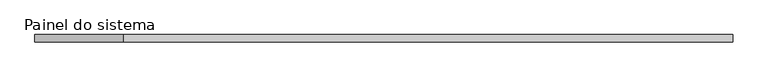
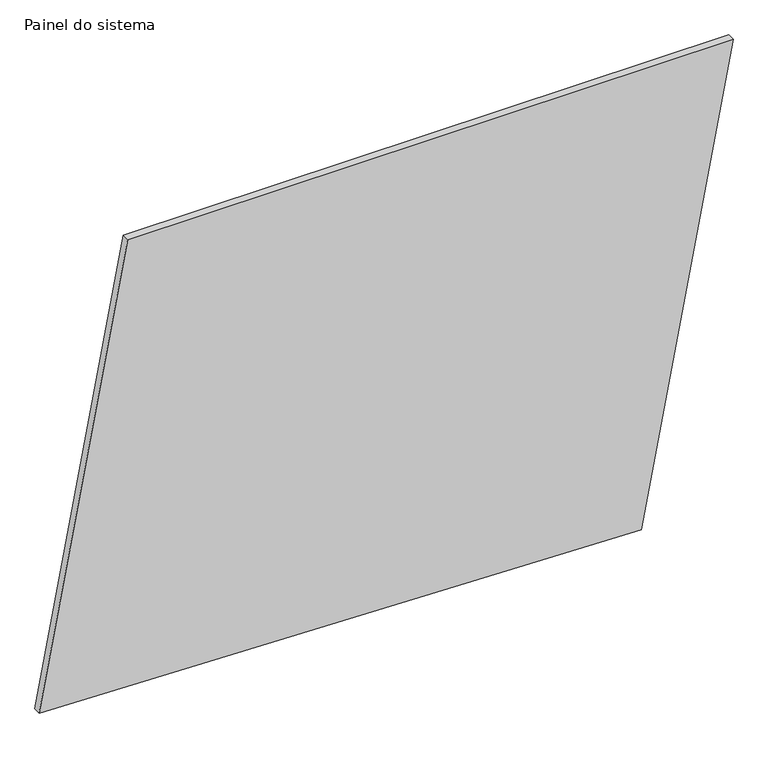
"""IFC4 building model written with IfcOpenShell, lengths in millimetres: plate geometry, Painel do sistema : Envidraçado."""

from ifc_helpers import new_model, si_unit, frame, origin, place, context, project, spatial, polyline, outline, extrude, source, transform, mapped, element, save


def painel_do_sistema_e6de913f(model_context):
    return source(origin(), model_context, "Body", "SweptSolid", [
        extrude(outline(polyline([(58.5472055, -1202.3440051), (0.0, 884.7575899), (1685.6103796, 1202.3440051), (1685.6103796, -895.7884885), (58.5472055, -1202.3440051)])), frame((0.0, 24.5, 0.0), z_axis=(0.0, 1.0, 0.0), x_axis=(0.0, 0.0, 1.0)), (0.0, 0.0, 1.0), 25.0),
    ])


if __name__ == "__main__":
    model = new_model("IFC4")
    model_context = context("Model", 3, world=origin())
    ifc_project = project(units=[si_unit("LENGTHUNIT", "METRE", prefix="MILLI")], contexts=[model_context])
    site = spatial("IfcSite", under=ifc_project)
    building = spatial("IfcBuilding", under=site)
    placement = place(None, origin())
    painel_do_sistema_shape = painel_do_sistema_e6de913f(model_context)
    element("IfcPlate", 1, ObjectType="Painel do sistema : Envidraçado", at=placement, inside=building, context=model_context, shape_type="MappedRepresentation", body=[
        mapped(painel_do_sistema_shape, transform((0.0, 0.0, 0.0), x_axis=(1.0, 0.0, 0.0), y_axis=(0.0, 1.0, 0.0), z_axis=(0.0, 0.0, 1.0))),
    ])
    save(model, "model.ifc")

# Revit data of these elements
# Type "Painel do sistema : Envidraçado"
#   Construction Type Id = "GSP4R"
#   Analytic Construction = "Vidraça única Pilkington 1/8 pol"
#   Visual Light Transmittance = 0.9
#   Solar Heat Gain Coefficient = 0.86
#   Heat Transfer Coefficient (U) = 6.7069 W/(m²·K)
# Element 1 (IfcPlate, "Painel do sistema : Envidraçado")
#   Materials on its faces: "Vidro"
# Materials
#   "Vidro": class "Vidro", colour RGB 0 128 192, transparency 0.9, Description = "Vidro de sílica", Cost = 0
